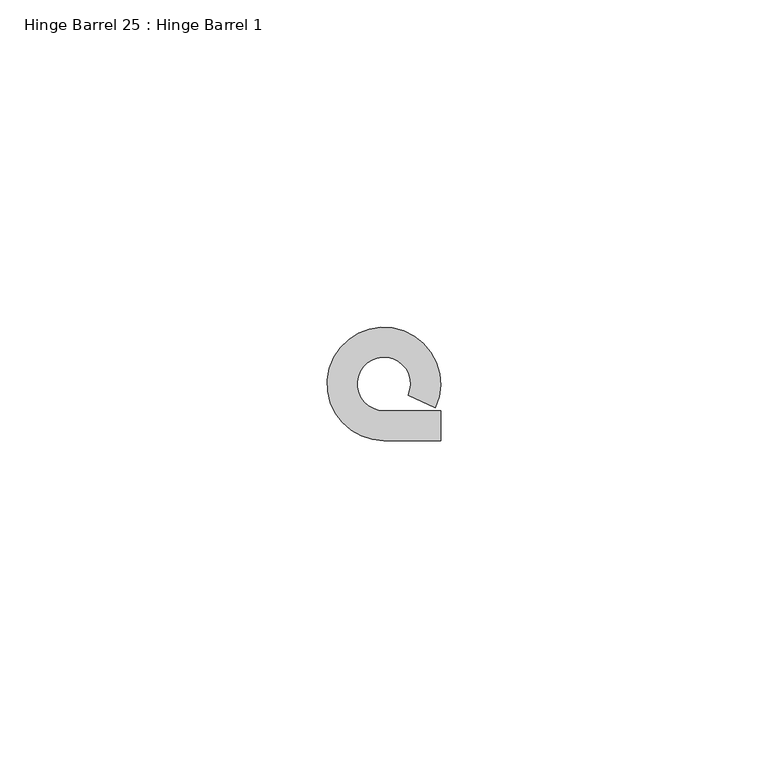
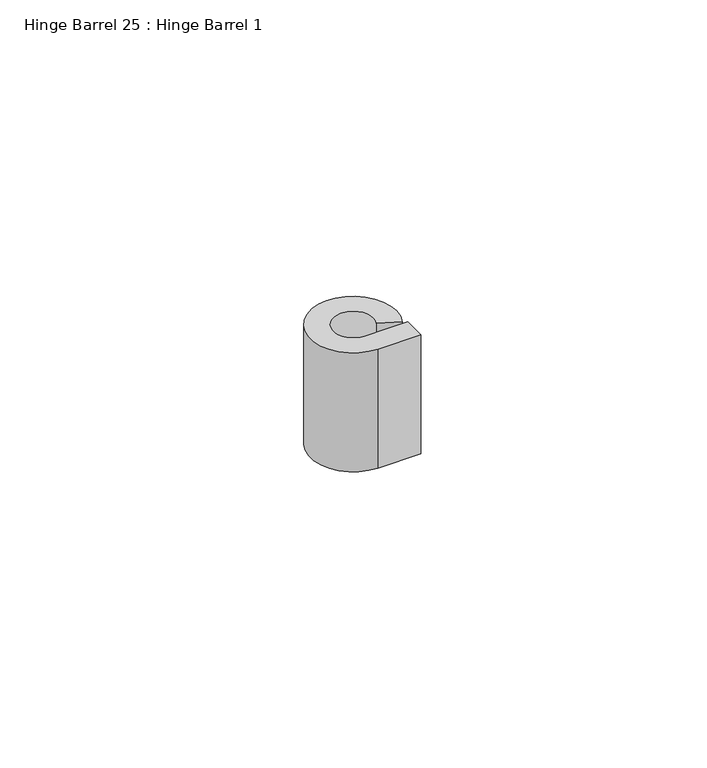
"""IFC4 building model written with IfcOpenShell, lengths in millimetres: proxy geometry, Hinge Barrel 25 : Hinge Barrel 1."""

from ifc_helpers import new_model, si_unit, point, frame, frame_2d, origin, place, context, project, spatial, polyline, circle_curve, trimmed, segment, composite_curve, outline, extrude, source, transform, mapped, element, save


def hinge_barrel_25_hinge_barrel_1_91723ac2(model_context):
    return source(origin(), model_context, "Body", "SweptSolid", [
        extrude(outline(composite_curve([segment(polyline([(587323.2214739, -531780.6943841), (587327.7934739, -531780.6943841), (587327.7934739, -531785.2584466), (587319.1320739, -531785.2584466)]), True, "CONTINUOUS"), segment(trimmed(circle_curve(frame_2d((587319.1320739, -531776.6049841)), 8.6534625), [point((587319.1320739, -531785.2584466))], [point((587326.986084, -531780.2377433))], False, "CARTESIAN"), True, "CONTINUOUS"), segment(polyline([(587326.986084, -531780.2377433), (587322.8436736, -531778.321731)]), True, "CONTINUOUS"), segment(trimmed(circle_curve(frame_2d((587319.1320739, -531776.6049841)), 4.0894), [point((587322.8436736, -531778.321731))], [point((587319.1320739, -531780.6943841))], True, "CARTESIAN"), True, "CONTINUOUS"), segment(polyline([(587319.1320739, -531780.6943841), (587323.2214739, -531780.6943841)]), True, "CONTINUOUS")], self_intersect=False)), frame((0.0, 0.0, 1123.95), z_axis=(0.0, 0.0, 1.0), x_axis=(1.0, 0.0, 0.0)), (0.0, 0.0, 1.0), 25.4),
    ])


if __name__ == "__main__":
    model = new_model("IFC4")
    model_context = context("Model", 3, world=origin())
    ifc_project = project(units=[si_unit("LENGTHUNIT", "METRE", prefix="MILLI")], contexts=[model_context])
    site = spatial("IfcSite", under=ifc_project)
    building = spatial("IfcBuilding", under=site)
    placement = place(None, origin())
    hinge_barrel_25_hinge_barrel_1_shape = hinge_barrel_25_hinge_barrel_1_91723ac2(model_context)
    element("IfcBuildingElementProxy", 1, Name="Hinge Barrel 25 : Hinge Barrel 1", ObjectType="Hinge Barrel 25 : Hinge Barrel 1", at=placement, inside=building, context=model_context, shape_type="MappedRepresentation", body=[
        mapped(hinge_barrel_25_hinge_barrel_1_shape, transform((0.0, 0.0, 0.0), x_axis=(1.0, 0.0, 0.0), y_axis=(0.0, 1.0, 0.0), z_axis=(0.0, 0.0, 1.0))),
    ])
    save(model, "model.ifc")

# Revit data of these elements
# Element 1 (IfcBuildingElementProxy, "Hinge Barrel 25 : Hinge Barrel 1")
#   Materials on its faces: "6\"X6\" WELD-ON STL BUTT HINGE"
# Materials
#   "6\"X6\" WELD-ON STL BUTT HINGE": class "Metal", colour RGB 189 187 185, transparency 0, Description = "Carbon steel", Cost = 0
